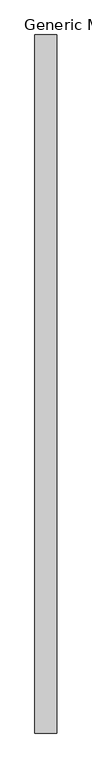
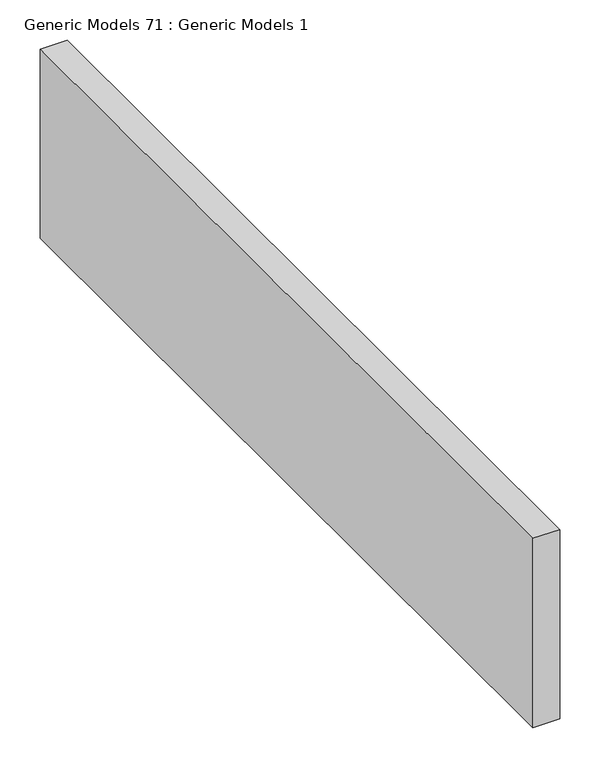
"""IFC4 building model written with IfcOpenShell, lengths in millimetres: proxy geometry, Generic Models 71 : Generic Models 1."""

import ifcopenshell
import ifcopenshell.guid

model = None  # the IFC model being written
_history = None  # IfcOwnerHistory: only IFC2X3 demands one
_inside = {}  # id of a spatial element -> (the spatial element, [elements in it])
_under = {}  # id of a project, library or spatial element -> (it, [spatial elements below it])
_declared = {}  # id of a project -> (the project, [libraries it declares])
_typed = {}  # id of a type object -> (the type object, [elements of that type])
_made_of = {}  # id of a material, layer set ... -> (it, [elements and type objects made of it])


def new_model(schema):
    """Start an empty IFC model of exactly this schema.

    Asked for "IFC4X3", IfcOpenShell would pick the latest addendum, in which some entities
    have other attributes; the version numbers below select the first issue.
    IFC2X3 requires an IfcOwnerHistory on every rooted entity: one is made here for all.
    """
    global model, _history
    if schema == "IFC4X3":
        model = ifcopenshell.file(schema_version=(4, 3, 0, 0))
    else:
        model = ifcopenshell.file(schema=schema)
    _inside.clear()
    _under.clear()
    _declared.clear()
    _typed.clear()
    _made_of.clear()
    _history = None
    if model.schema == "IFC2X3":
        org = make("IfcOrganization", Name="unknown")
        user = make(
            "IfcPersonAndOrganization",
            ThePerson=make("IfcPerson", FamilyName="unknown"),
            TheOrganization=org,
        )
        app = make(
            "IfcApplication",
            ApplicationDeveloper=org,
            Version="unknown",
            ApplicationFullName="unknown",
            ApplicationIdentifier="unknown",
        )
        _history = make(
            "IfcOwnerHistory",
            OwningUser=user,
            OwningApplication=app,
            ChangeAction="ADDED",
            CreationDate=0,
        )
    return model


def make(cls, **values):
    """One entity of the class cls with the attributes given. An attribute that is None is left unset."""
    return model.create_entity(
        cls, **{name: value for name, value in values.items() if value is not None}
    )


def rooted(cls, **values):
    """An entity with a GlobalId (a new one), such as an element, a storey or a relation."""
    return make(cls, GlobalId=ifcopenshell.guid.new(), OwnerHistory=_history, **values)


def si_unit(unit_type, name, prefix=None):
    """IfcSIUnit, for example si_unit("LENGTHUNIT", "METRE", prefix="MILLI")."""
    return make("IfcSIUnit", UnitType=unit_type, Prefix=prefix, Name=name)


def assignment(units):
    """IfcUnitAssignment: the units of a project."""
    return None if units is None else make("IfcUnitAssignment", Units=units)


def point(xyz):
    """IfcCartesianPoint."""
    return None if xyz is None else make("IfcCartesianPoint", Coordinates=xyz)


def direction(xyz):
    """IfcDirection."""
    return None if xyz is None else make("IfcDirection", DirectionRatios=xyz)


def frame(location, z_axis=None, x_axis=None):
    """IfcAxis2Placement3D, a coordinate frame: its origin and axes. An axis left out is left unset."""
    return make(
        "IfcAxis2Placement3D",
        Location=point(location),
        Axis=direction(z_axis),
        RefDirection=direction(x_axis),
    )


def origin():
    """The frame at (0, 0, 0) with its axes left unset."""
    return frame((0.0, 0.0, 0.0))


def place(relative_to, where):
    """IfcLocalPlacement: puts the frame where relative to a parent placement (None: the world)."""
    return make(
        "IfcLocalPlacement", PlacementRelTo=relative_to, RelativePlacement=where
    )


def context(
    kind, dimensions, precision=None, world=None, true_north=None, identifier=None
):
    """IfcGeometricRepresentationContext, for example the 3D "Model" context."""
    return make(
        "IfcGeometricRepresentationContext",
        ContextIdentifier=identifier,
        ContextType=kind,
        CoordinateSpaceDimension=dimensions,
        Precision=precision,
        WorldCoordinateSystem=world,
        TrueNorth=true_north,
    )


def project(units=None, contexts=None):
    """IfcProject with its units and contexts."""
    return rooted(
        "IfcProject",
        Name="project",
        RepresentationContexts=contexts,
        UnitsInContext=assignment(units),
    )


def spatial(cls, under=None, at=None, **own):
    """A site, building, storey or space (cls), placed at a placement, below another one or the project."""
    s = rooted(cls, ObjectPlacement=at, **own)
    if under is not None:
        _under.setdefault(under.id(), (under, []))[1].append(s)
    return s


def polyline(points):
    """IfcPolyline through the points."""
    return make("IfcPolyline", Points=[point(p) for p in points])


def outline(outer, holes=None, kind="AREA"):
    """IfcArbitraryClosedProfileDef: a profile drawn as a closed curve; with holes, ...WithVoids."""
    if holes is None:
        return make("IfcArbitraryClosedProfileDef", ProfileType=kind, OuterCurve=outer)
    return make(
        "IfcArbitraryProfileDefWithVoids",
        ProfileType=kind,
        OuterCurve=outer,
        InnerCurves=holes,
    )


def extrude(swept, where, along, depth):
    """IfcExtrudedAreaSolid: the profile swept, set in the frame where, extruded along a direction by depth."""
    return make(
        "IfcExtrudedAreaSolid",
        SweptArea=swept,
        Position=where,
        ExtrudedDirection=direction(along),
        Depth=depth,
    )


def shape(context_of_items, identifier, shape_type, items):
    """IfcShapeRepresentation: the items that make up one representation, for example the "Body"."""
    return make(
        "IfcShapeRepresentation",
        ContextOfItems=context_of_items,
        RepresentationIdentifier=identifier,
        RepresentationType=shape_type,
        Items=items,
    )


def source(mapping_origin, context_of_items, identifier, shape_type, items):
    """IfcRepresentationMap: a shape defined once, which mapped items show again and again."""
    return make(
        "IfcRepresentationMap",
        MappingOrigin=mapping_origin,
        MappedRepresentation=shape(context_of_items, identifier, shape_type, items),
    )


def transform(
    local_origin,
    x_axis=None,
    y_axis=None,
    z_axis=None,
    scale=None,
    scale2=None,
    scale3=None,
    uniform=True,
):
    """IfcCartesianTransformationOperator3D, or its non-uniform kind. x_axis, y_axis, z_axis: its Axis1, 2, 3."""
    if uniform:
        return make(
            "IfcCartesianTransformationOperator3D",
            Axis1=direction(x_axis),
            Axis2=direction(y_axis),
            LocalOrigin=point(local_origin),
            Scale=scale,
            Axis3=direction(z_axis),
        )
    return make(
        "IfcCartesianTransformationOperator3DnonUniform",
        Axis1=direction(x_axis),
        Axis2=direction(y_axis),
        LocalOrigin=point(local_origin),
        Scale=scale,
        Axis3=direction(z_axis),
        Scale2=scale2,
        Scale3=scale3,
    )


def mapped(mapping_source, mapping_target):
    """IfcMappedItem: shows the shape of a source again, moved by a transform."""
    return make(
        "IfcMappedItem", MappingSource=mapping_source, MappingTarget=mapping_target
    )


def made_of(thing, what):
    """Note that an element or type object is made of a material, layer set ...; save() writes the relation."""
    if what is not None:
        _made_of.setdefault(what.id(), (what, []))[1].append(thing)
    return thing


def element(
    cls,
    number,
    at=None,
    inside=None,
    cuts=None,
    type_object=None,
    material=None,
    context=None,
    identifier="Body",
    shape_type=None,
    held_by="IfcProductDefinitionShape",
    body=None,
    shapes=None,
    **own,
):
    """One element of the class cls, such as IfcWall. Its Tag is "e" and its number.

    at: its placement. inside: the storey or other place that contains it. cuts: it is an
    opening in that element (IfcRelVoidsElement). A single representation is given by context,
    identifier, shape_type and body (its items); several are given by shapes. held_by: the class
    of the entity that holds the representations. save() writes the other relations.
    """
    e = rooted(cls, Tag="e%d" % number, ObjectPlacement=at, **own)
    if body is not None:
        shapes = [shape(context, identifier, shape_type, body)]
    if shapes is not None:
        e.Representation = make(held_by, Representations=shapes)
    if inside is not None:
        _inside.setdefault(inside.id(), (inside, []))[1].append(e)
    if cuts is not None:
        rooted(
            "IfcRelVoidsElement", RelatingBuildingElement=cuts, RelatedOpeningElement=e
        )
    if type_object is not None:
        _typed.setdefault(type_object.id(), (type_object, []))[1].append(e)
    return made_of(e, material)


def aggregate(whole, parts):
    """IfcRelAggregates: a whole, such as a stair, and the parts it consists of."""
    return rooted("IfcRelAggregates", RelatingObject=whole, RelatedObjects=parts)


def save(model, path):
    """Write the relations noted so far, then the file.

    IfcRelAggregates (storeys below a building ...), IfcRelContainedInSpatialStructure (elements
    in a storey), IfcRelDefinesByType, IfcRelAssociatesMaterial and IfcRelDeclares: one each for
    every whole, place, type object, material and project.
    """
    for whole, parts in _under.values():
        aggregate(whole, parts)
    for where, things in _inside.values():
        rooted(
            "IfcRelContainedInSpatialStructure",
            RelatedElements=things,
            RelatingStructure=where,
        )
    for kind, things in _typed.values():
        rooted("IfcRelDefinesByType", RelatedObjects=things, RelatingType=kind)
    for what, things in _made_of.values():
        rooted("IfcRelAssociatesMaterial", RelatedObjects=things, RelatingMaterial=what)
    for by, libraries in _declared.values():
        rooted("IfcRelDeclares", RelatingContext=by, RelatedDefinitions=libraries)
    model.write(path)


def generic_models_71_generic_models_1_508a995f(model_context):
    return source(origin(), model_context, "Body", "SweptSolid", [
        extrude(outline(polyline([(50952.4, 0.0), (50914.3, 0.0), (50914.3, 1219.2), (50952.4, 1219.2), (50952.4, 0.0)])), frame((0.0, 0.0, 5222.478125), z_axis=(0.0, 0.0, 1.0), x_axis=(1.0, 0.0, 0.0)), (0.0, 0.0, 1.0), 285.75),
    ])


if __name__ == "__main__":
    model = new_model("IFC4")
    model_context = context("Model", 3, world=origin())
    ifc_project = project(units=[si_unit("LENGTHUNIT", "METRE", prefix="MILLI")], contexts=[model_context])
    site = spatial("IfcSite", under=ifc_project)
    building = spatial("IfcBuilding", under=site)
    placement = place(None, origin())
    generic_models_71_generic_models_1_shape = generic_models_71_generic_models_1_508a995f(model_context)
    element("IfcBuildingElementProxy", 1, Name="Generic Models 71 : Generic Models 1", ObjectType="Generic Models 71 : Generic Models 1", at=placement, inside=building, context=model_context, shape_type="MappedRepresentation", body=[
        mapped(generic_models_71_generic_models_1_shape, transform((0.0, 0.0, 0.0), x_axis=(1.0, 0.0, 0.0), y_axis=(0.0, 1.0, 0.0), z_axis=(0.0, 0.0, 1.0))),
    ])
    save(model, "model.ifc")

# Revit data of these elements
# Element 1 (IfcBuildingElementProxy, "Generic Models 71 : Generic Models 1")
#   Materials on its faces: "DOUBLE 2X WOOD TOP PLATE"
# Materials
#   "DOUBLE 2X WOOD TOP PLATE": class "Wood", colour RGB 234 198 147, transparency 0, Description = "Pinus Echinata", Cost = 0
